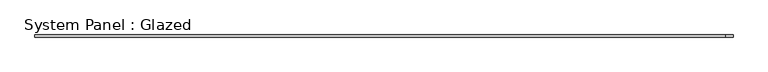
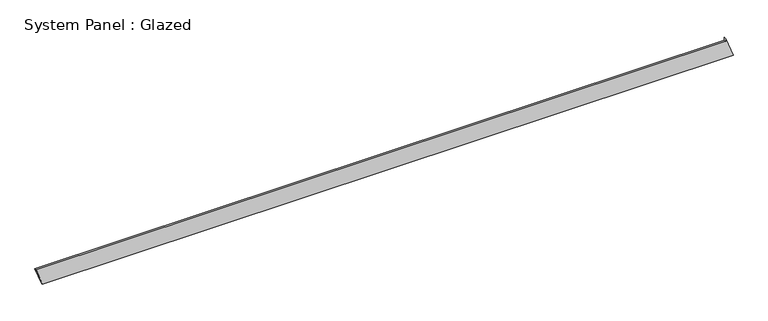
"""IFC4 building model written with IfcOpenShell, lengths in millimetres: plate geometry, System Panel : Glazed."""

from ifc_helpers import new_model, si_unit, frame, origin, place, context, project, spatial, polyline, outline, extrude, source, transform, mapped, element, save


def system_panel_glazed_701bf6f3(model_context):
    return source(origin(), model_context, "Body", "SweptSolid", [
        extrude(outline(polyline([(0.0, -3964.1196538), (0.0, 4035.4320594), (234.126736, 3950.0305658), (198.7713971, 3950.02827), (199.28994, -4035.4320594), (0.0, -3964.1196538)])), frame((0.0, -49.5, 0.0), z_axis=(0.0, 1.0, 0.0), x_axis=(0.0, 0.0, 1.0)), (0.0, 0.0, 1.0), 25.0),
    ])


if __name__ == "__main__":
    model = new_model("IFC4")
    model_context = context("Model", 3, world=origin())
    ifc_project = project(units=[si_unit("LENGTHUNIT", "METRE", prefix="MILLI")], contexts=[model_context])
    site = spatial("IfcSite", under=ifc_project)
    building = spatial("IfcBuilding", under=site)
    placement = place(None, origin())
    system_panel_glazed_shape = system_panel_glazed_701bf6f3(model_context)
    element("IfcPlate", 1, ObjectType="System Panel : Glazed", at=placement, inside=building, context=model_context, shape_type="MappedRepresentation", body=[
        mapped(system_panel_glazed_shape, transform((0.0, 0.0, 0.0), x_axis=(1.0, 0.0, 0.0), y_axis=(0.0, 1.0, 0.0), z_axis=(0.0, 0.0, 1.0))),
    ])
    save(model, "model.ifc")

# Revit data of these elements
# Element 1 (IfcPlate, "System Panel : Glazed")
#   Materials on its faces: "Glass"
# Materials
#   "Glass": class "Glass", colour RGB 218 227 224, transparency 0.85, Description = "Soda Lime Glass", Cost = 0
